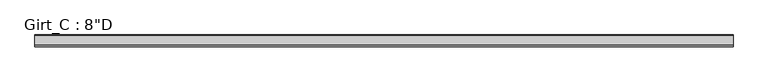
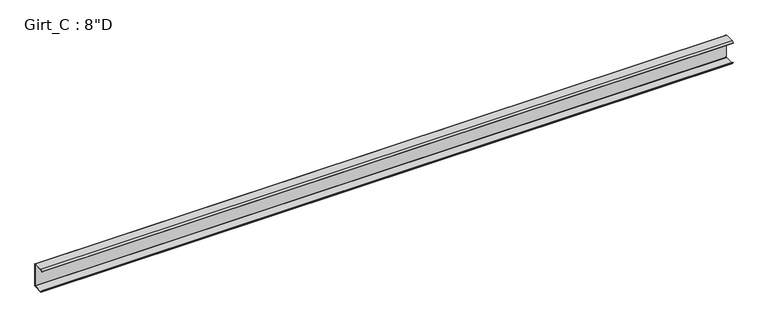
"""IFC4 building model written with IfcOpenShell, lengths in millimetres: beam geometry."""

from ifc_helpers import new_model, si_unit, point, frame, frame_2d, origin, place, context, project, spatial, polyline, circle_curve, trimmed, segment, composite_curve, outline, extrude, source, transform, mapped, element, save


def beam_6fd188a8(model_context):
    return source(origin(), model_context, "Body", "SweptSolid", [
        extrude(outline(composite_curve([segment(polyline([(-87.5109375, 101.6), (-3.3734375, 101.6)]), True, "CONTINUOUS"), segment(trimmed(circle_curve(frame_2d((-3.3734375, 96.8375)), 4.7625), [point((-3.3734375, 101.6))], [point((1.3890625, 96.8375))], False, "CARTESIAN"), True, "CONTINUOUS"), segment(polyline([(1.3890625, 96.8375), (1.3890625, -96.8375)]), True, "CONTINUOUS"), segment(trimmed(circle_curve(frame_2d((-3.3734375, -96.8375)), 4.7625), [point((1.3890625, -96.8375))], [point((-3.3734375, -101.6))], False, "CARTESIAN"), True, "CONTINUOUS"), segment(polyline([(-3.3734375, -101.6), (-87.5109375, -101.6), (-99.7792647, -86.979177), (-97.6510975, -85.1934327), (-86.2154765, -98.821875), (-3.2694106, -98.821875)]), True, "CONTINUOUS"), segment(trimmed(circle_curve(frame_2d((-3.3748024, -96.8389339)), 1.9857399), [point((-3.2694106, -98.821875))], [point((-1.3890625, -96.8389339))], True, "CARTESIAN"), True, "CONTINUOUS"), segment(polyline([(-1.3890625, -96.8389339), (-1.3890625, 96.8381931)]), True, "CONTINUOUS"), segment(trimmed(circle_curve(frame_2d((-3.3741066, 96.8381931)), 1.9850441), [point((-1.3890625, 96.8381931))], [point((-3.3005807, 98.821875))], True, "CARTESIAN"), True, "CONTINUOUS"), segment(polyline([(-3.3005807, 98.821875), (-86.2154765, 98.821875), (-97.6278742, 85.221109), (-99.7560415, 87.0068534), (-87.5109375, 101.6)]), True, "CONTINUOUS")], self_intersect=False)), frame((-3051.175, 0.0, 0.0), z_axis=(1.0, 0.0, 0.0), x_axis=(0.0, 1.0, 0.0)), (0.0, 0.0, 1.0), 5864.225),
    ])


if __name__ == "__main__":
    model = new_model("IFC4")
    model_context = context("Model", 3, world=origin())
    ifc_project = project(units=[si_unit("LENGTHUNIT", "METRE", prefix="MILLI")], contexts=[model_context])
    site = spatial("IfcSite", under=ifc_project)
    building = spatial("IfcBuilding", under=site)
    placement = place(None, origin())
    beam_shape = beam_6fd188a8(model_context)
    element("IfcBeam", 1, ObjectType="Girt_C : 8\"D", at=placement, inside=building, context=model_context, shape_type="MappedRepresentation", body=[
        mapped(beam_shape, transform((0.0, 0.0, 0.0), x_axis=(1.0, 0.0, 0.0), y_axis=(0.0, 1.0, 0.0), z_axis=(0.0, 0.0, 1.0))),
    ])
    save(model, "model.ifc")

# Revit data of these elements
# Type "Girt_C : 8\"D"
#   half leg = 0' - 1 3/4"
#   Web_Thickness = 0' - 0 7/64"
#   Length [instance default] = 10' - 0"
#   Leg_1 = 0' - 3 1/2"
#   Height = 0' - 8"
#   Structural Material [instance default] = none
# Element 1 (IfcBeam, "Girt_C : 8\"D")
#   Structural Material = CEE' SECTION (8.0x3.5C - SEE STRUCT. DWGS)
#   Materials on its faces: "CEE' SECTION (8.0x3.5C - SEE STRUCT. DWGS)"
# Materials
#   "CEE' SECTION (8.0x3.5C - SEE STRUCT. DWGS)": class "Metal", colour RGB 137 146 153, transparency 0, Description = "Steel, mill finish", Cost = 0
